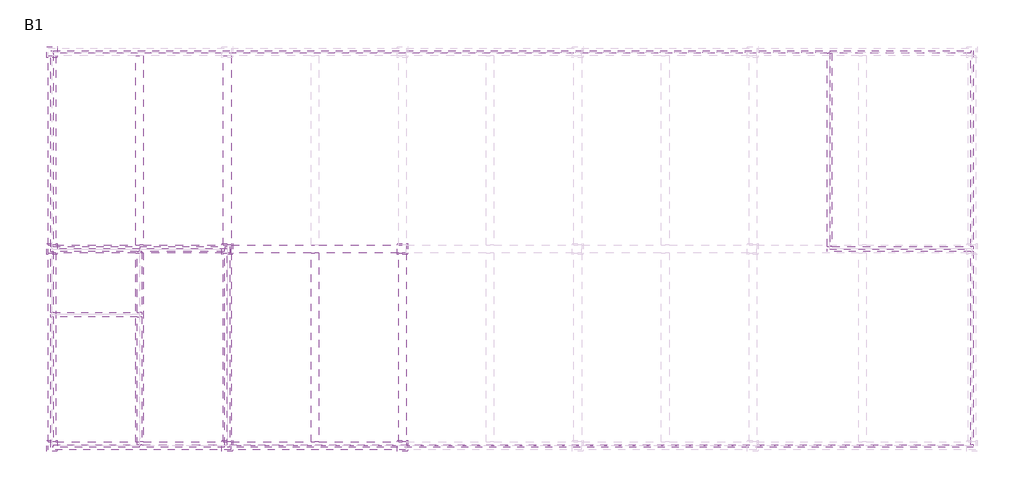
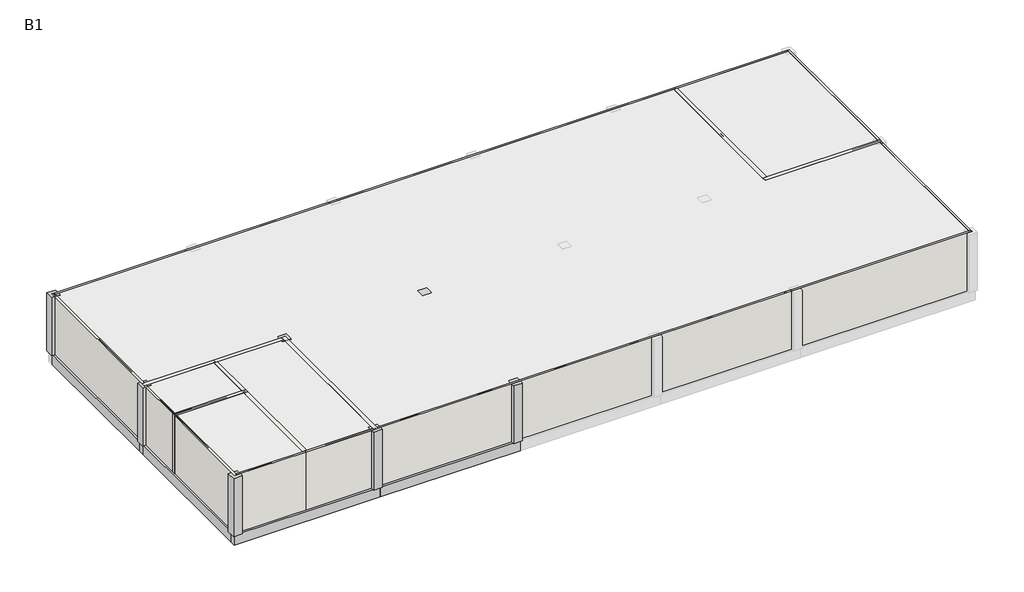
# One storey, part 1 of 2: 18 walls, 12 beams, 7 columns, 5 slabs.
"""IFC4 building model written with IfcOpenShell, lengths in millimetres."""

from ifc_helpers import new_model, si_unit, frame, origin, origin_with_axes, place, context, project, spatial, polyline, outline, extrude, faceted_brep, element, save

model = new_model("IFC4")

# Units and contexts
model_context = context("Model", 3, world=origin())
ifc_project = project(units=[si_unit("LENGTHUNIT", "METRE", prefix="MILLI")], contexts=[model_context])

# Site, building, storey
site = spatial("IfcSite", under=ifc_project)
building = spatial("IfcBuilding", under=site)
storey = spatial("IfcBuildingStorey", under=building, Name="B1", Elevation=-4000.0)

# Beams
placement = place(None, origin())
element("IfcBeam", 1, ObjectType="Concrete-Rectangular-Beam : BM111_400x500_RG1", at=placement, inside=storey, context=model_context, shape_type="SweptSolid", body=[
    extrude(outline(polyline([(49284.6521483, 181748.8614395), (49634.6521483, 181748.8614395), (49634.6521483, 173098.8614395), (49284.6521483, 173098.8614395), (49284.6521483, 181748.8614395)])), frame((0.0, 0.0, -600.0), z_axis=(0.0, 0.0, 1.0), x_axis=(1.0, 0.0, 0.0)), (0.0, 0.0, 1.0), 600.0),
])
element("IfcBeam", 2, ObjectType="Concrete-Rectangular-Beam : BM111_400x500_RG1", at=placement, inside=storey, context=model_context, shape_type="SweptSolid", body=[
    extrude(outline(polyline([(49284.6521483, 172748.8614395), (49634.6521483, 172748.8614395), (49634.6521483, 164098.8614395), (49284.6521483, 164098.8614395), (49284.6521483, 172748.8614395)])), frame((0.0, 0.0, -600.0), z_axis=(0.0, 0.0, 1.0), x_axis=(1.0, 0.0, 0.0)), (0.0, 0.0, 1.0), 600.0),
])
element("IfcBeam", 3, ObjectType="Concrete-Rectangular-Beam : BM111_400x500_RG1", at=placement, inside=storey, context=model_context, shape_type="SweptSolid", body=[
    extrude(outline(polyline([(57284.6521483, 172748.8614395), (57634.6521483, 172748.8614395), (57634.6521483, 164098.8614395), (57284.6521483, 164098.8614395), (57284.6521483, 172748.8614395)])), frame((0.0, 0.0, -600.0), z_axis=(0.0, 0.0, 1.0), x_axis=(1.0, 0.0, 0.0)), (0.0, 0.0, 1.0), 600.0),
])
element("IfcBeam", 4, ObjectType="Concrete-Rectangular-Beam : BM111_400x500_RG1", at=placement, inside=storey, context=model_context, shape_type="Brep", body=[
    faceted_brep([(53634.6521483, 172748.8614395, 0.0), (53634.6521483, 173098.8614395, 0.0), (53284.6521483, 173098.8614395, 0.0), (49634.6521483, 173098.8614395, 0.0), (49284.6521483, 173098.8614395, 0.0), (45634.6521483, 173098.8614395, 0.0), (45284.6521483, 173098.8614395, 0.0), (45284.6521483, 172748.8614395, 0.0), (45634.6521483, 172748.8614395, 0.0), (49284.6521483, 172748.8614395, 0.0), (49634.6521483, 172748.8614395, 0.0), (53284.6521483, 172748.8614395, 0.0), (53634.6521483, 172748.8614395, -600.0), (45284.6521483, 172748.8614395, -600.0), (45634.6521483, 172748.8614395, -600.0), (49284.6521483, 172748.8614395, -600.0), (49634.6521483, 172748.8614395, -600.0), (53284.6521483, 172748.8614395, -600.0), (53634.6521483, 173098.8614395, -600.0), (45284.6521483, 173098.8614395, -600.0), (45634.6521483, 173098.8614395, -600.0), (49284.6521483, 173098.8614395, -600.0), (49634.6521483, 173098.8614395, -600.0), (53284.6521483, 173098.8614395, -600.0)], [[[0, 1, 2, 3, 4, 5, 6, 7, 8, 9, 10, 11]], [[12, 0, 11, 10, 9, 8, 7, 13, 14, 15, 16, 17]], [[18, 12, 17, 16, 15, 14, 13, 19, 20, 21, 22, 23]], [[1, 18, 23, 22, 21, 20, 19, 6, 5, 4, 3, 2]], [[1, 0, 12, 18]], [[7, 6, 19, 13]]]),
])
element("IfcBeam", 5, ObjectType="Concrete-Rectangular-Beam : BM111_400x500_RG1", at=placement, inside=storey, context=model_context, shape_type="Brep", body=[
    faceted_brep([(61634.6521483, 172748.8614395, 0.0), (61634.6521483, 173098.8614395, 0.0), (61284.6521483, 173098.8614395, 0.0), (57634.6521483, 173098.8614395, 0.0), (57284.6521483, 173098.8614395, 0.0), (53634.6521483, 173098.8614395, 0.0), (53634.6521483, 172748.8614395, 0.0), (57284.6521483, 172748.8614395, 0.0), (57634.6521483, 172748.8614395, 0.0), (61284.6521483, 172748.8614395, 0.0), (61634.6521483, 172748.8614395, -600.0), (53634.6521483, 172748.8614395, -600.0), (57284.6521483, 172748.8614395, -600.0), (57634.6521483, 172748.8614395, -600.0), (61284.6521483, 172748.8614395, -600.0), (61634.6521483, 173098.8614395, -600.0), (53634.6521483, 173098.8614395, -600.0), (57284.6521483, 173098.8614395, -600.0), (57634.6521483, 173098.8614395, -600.0), (61284.6521483, 173098.8614395, -600.0)], [[[0, 1, 2, 3, 4, 5, 6, 7, 8, 9]], [[10, 0, 9, 8, 7, 6, 11, 12, 13, 14]], [[15, 10, 14, 13, 12, 11, 16, 17, 18, 19]], [[1, 15, 19, 18, 17, 16, 5, 4, 3, 2]], [[1, 0, 10, 15]], [[6, 5, 16, 11]]]),
])
element("IfcBeam", 6, ObjectType="Concrete-Rectangular-Beam : BM111_400x500_RG1", at=placement, inside=storey, context=model_context, shape_type="Brep", body=[
    faceted_brep([(53634.6521483, 163748.8614395, 0.0), (53634.6521483, 164098.8614395, 0.0), (53284.6521483, 164098.8614395, 0.0), (49634.6521483, 164098.8614395, 0.0), (49284.6521483, 164098.8614395, 0.0), (45634.6521483, 164098.8614395, 0.0), (45284.6521483, 164098.8614395, 0.0), (45284.6521483, 163748.8614395, 0.0), (53634.6521483, 163748.8614395, -600.0), (45284.6521483, 163748.8614395, -600.0), (53634.6521483, 164098.8614395, -600.0), (45284.6521483, 164098.8614395, -600.0), (45634.6521483, 164098.8614395, -600.0), (49284.6521483, 164098.8614395, -600.0), (49634.6521483, 164098.8614395, -600.0), (53284.6521483, 164098.8614395, -600.0)], [[[0, 1, 2, 3, 4, 5, 6, 7]], [[8, 0, 7, 9]], [[10, 8, 9, 11, 12, 13, 14, 15]], [[1, 10, 15, 14, 13, 12, 11, 6, 5, 4, 3, 2]], [[1, 0, 8, 10]], [[7, 6, 11, 9]]]),
])
element("IfcBeam", 7, ObjectType="Concrete-Rectangular-Beam : BM111_400x500_RG1", at=placement, inside=storey, context=model_context, shape_type="Brep", body=[
    faceted_brep([(61634.6521483, 163748.8614395, 0.0), (61634.6521483, 164098.8614395, 0.0), (61284.6521483, 164098.8614395, 0.0), (57634.6521483, 164098.8614395, 0.0), (57284.6521483, 164098.8614395, 0.0), (53634.6521483, 164098.8614395, 0.0), (53634.6521483, 163748.8614395, 0.0), (61634.6521483, 163748.8614395, -600.0), (53634.6521483, 163748.8614395, -600.0), (61634.6521483, 164098.8614395, -600.0), (53634.6521483, 164098.8614395, -600.0), (57284.6521483, 164098.8614395, -600.0), (57634.6521483, 164098.8614395, -600.0), (61284.6521483, 164098.8614395, -600.0)], [[[0, 1, 2, 3, 4, 5, 6]], [[7, 0, 6, 8]], [[9, 7, 8, 10, 11, 12, 13]], [[1, 9, 13, 12, 11, 10, 5, 4, 3, 2]], [[1, 0, 7, 9]], [[6, 5, 10, 8]]]),
])
element("IfcBeam", 8, ObjectType="Concrete-Rectangular-Beam : BM111_400x500_RG1", at=placement, inside=storey, context=model_context, shape_type="SweptSolid", body=[
    extrude(outline(polyline([(45284.6521483, 181748.8614395), (45634.6521483, 181748.8614395), (45634.6521483, 173098.8614395), (45284.6521483, 173098.8614395), (45284.6521483, 181748.8614395)])), frame((0.0, 0.0, -600.0), z_axis=(0.0, 0.0, 1.0), x_axis=(1.0, 0.0, 0.0)), (0.0, 0.0, 1.0), 600.0),
])
element("IfcBeam", 9, ObjectType="Concrete-Rectangular-Beam : BM111_400x500_RG1", at=placement, inside=storey, context=model_context, shape_type="SweptSolid", body=[
    extrude(outline(polyline([(45284.6521483, 172748.8614395), (45634.6521483, 172748.8614395), (45634.6521483, 164098.8614395), (45284.6521483, 164098.8614395), (45284.6521483, 172748.8614395)])), frame((0.0, 0.0, -600.0), z_axis=(0.0, 0.0, 1.0), x_axis=(1.0, 0.0, 0.0)), (0.0, 0.0, 1.0), 600.0),
])
element("IfcBeam", 10, ObjectType="Concrete-Rectangular-Beam : BM111_400x500_RG1", at=placement, inside=storey, context=model_context, shape_type="SweptSolid", body=[
    extrude(outline(polyline([(53284.6521483, 181748.8614395), (53634.6521483, 181748.8614395), (53634.6521483, 173098.8614395), (53284.6521483, 173098.8614395), (53284.6521483, 181748.8614395)])), frame((0.0, 0.0, -600.0), z_axis=(0.0, 0.0, 1.0), x_axis=(1.0, 0.0, 0.0)), (0.0, 0.0, 1.0), 600.0),
])
element("IfcBeam", 11, ObjectType="Concrete-Rectangular-Beam : BM111_400x500_RG1", at=placement, inside=storey, context=model_context, shape_type="SweptSolid", body=[
    extrude(outline(polyline([(53284.6521483, 172748.8614395), (53634.6521483, 172748.8614395), (53634.6521483, 164098.8614395), (53284.6521483, 164098.8614395), (53284.6521483, 172748.8614395)])), frame((0.0, 0.0, -600.0), z_axis=(0.0, 0.0, 1.0), x_axis=(1.0, 0.0, 0.0)), (0.0, 0.0, 1.0), 600.0),
])
element("IfcBeam", 12, ObjectType="Concrete-Rectangular-Beam : BM111_400x500_RG1", at=placement, inside=storey, context=model_context, shape_type="SweptSolid", body=[
    extrude(outline(polyline([(61284.6521483, 172748.8614395), (61634.6521483, 172748.8614395), (61634.6521483, 164098.8614395), (61284.6521483, 164098.8614395), (61284.6521483, 172748.8614395)])), frame((0.0, 0.0, -600.0), z_axis=(0.0, 0.0, 1.0), x_axis=(1.0, 0.0, 0.0)), (0.0, 0.0, 1.0), 600.0),
])

# Columns
element("IfcColumn", 13, ObjectType="Concrete-Rectangular-Column : CL111_500x500", at=placement, inside=storey, context=model_context, shape_type="Brep", body=[
    faceted_brep([(45709.6521483, 182173.8614395, 0.0), (45709.6521483, 181673.8614395, 0.0), (45209.6521483, 181673.8614395, 0.0), (45209.6521483, 182173.8614395, 0.0), (45709.6521483, 182173.8614395, 3500.0), (45709.6521483, 182098.8614395, 3500.0), (45709.6521483, 181748.8614395, 3500.0), (45709.6521483, 181673.8614395, 3500.0), (45634.6521483, 181673.8614395, 3500.0), (45284.6521483, 181673.8614395, 3500.0), (45209.6521483, 181673.8614395, 3500.0), (45209.6521483, 182173.8614395, 3500.0)], [[[0, 1, 2, 3]], [[4, 5, 6, 7, 1, 0]], [[7, 8, 9, 10, 2, 1]], [[10, 11, 3, 2]], [[11, 4, 0, 3]], [[4, 11, 10, 9, 8, 7, 6, 5]]]),
])
element("IfcColumn", 14, ObjectType="Concrete-Rectangular-Column : CL111_500x500", at=placement, inside=storey, context=model_context, shape_type="Brep", body=[
    faceted_brep([(45709.6521483, 173173.8614395, 0.0), (45709.6521483, 172673.8614395, 0.0), (45209.6521483, 172673.8614395, 0.0), (45209.6521483, 173173.8614395, 0.0), (45709.6521483, 173173.8614395, 3500.0), (45709.6521483, 173098.8614395, 3500.0), (45709.6521483, 172748.8614395, 3500.0), (45709.6521483, 172673.8614395, 3500.0), (45634.6521483, 172673.8614395, 3500.0), (45284.6521483, 172673.8614395, 3500.0), (45209.6521483, 172673.8614395, 3500.0), (45209.6521483, 173173.8614395, 3500.0), (45284.6521483, 173173.8614395, 3500.0), (45634.6521483, 173173.8614395, 3500.0)], [[[0, 1, 2, 3]], [[4, 5, 6, 7, 1, 0]], [[7, 8, 9, 10, 2, 1]], [[10, 11, 3, 2]], [[11, 12, 13, 4, 0, 3]], [[4, 13, 12, 11, 10, 9, 8, 7, 6, 5]]]),
])
element("IfcColumn", 15, ObjectType="Concrete-Rectangular-Column : CL111_500x500", at=placement, inside=storey, context=model_context, shape_type="Brep", body=[
    faceted_brep([(53709.6521483, 173173.8614395, 0.0), (53709.6521483, 172673.8614395, 0.0), (53209.6521483, 172673.8614395, 0.0), (53209.6521483, 173173.8614395, 0.0), (53709.6521483, 173173.8614395, 3500.0), (53709.6521483, 173098.8614395, 3500.0), (53709.6521483, 172748.8614395, 3500.0), (53709.6521483, 172673.8614395, 3500.0), (53634.6521483, 172673.8614395, 3500.0), (53284.6521483, 172673.8614395, 3500.0), (53209.6521483, 172673.8614395, 3500.0), (53209.6521483, 172748.8614395, 3500.0), (53209.6521483, 173098.8614395, 3500.0), (53209.6521483, 173173.8614395, 3500.0), (53284.6521483, 173173.8614395, 3500.0), (53634.6521483, 173173.8614395, 3500.0)], [[[0, 1, 2, 3]], [[4, 5, 6, 7, 1, 0]], [[7, 8, 9, 10, 2, 1]], [[10, 11, 12, 13, 3, 2]], [[13, 14, 15, 4, 0, 3]], [[4, 15, 14, 13, 12, 11, 10, 9, 8, 7, 6, 5]]]),
])
element("IfcColumn", 16, ObjectType="Concrete-Rectangular-Column : CL111_500x500", at=placement, inside=storey, context=model_context, shape_type="Brep", body=[
    faceted_brep([(61709.6521483, 173173.8614395, 0.0), (61709.6521483, 172673.8614395, 0.0), (61209.6521483, 172673.8614395, 0.0), (61209.6521483, 173173.8614395, 0.0), (61709.6521483, 173173.8614395, 3500.0), (61709.6521483, 173098.8614395, 3500.0), (61709.6521483, 172748.8614395, 3500.0), (61709.6521483, 172673.8614395, 3500.0), (61634.6521483, 172673.8614395, 3500.0), (61284.6521483, 172673.8614395, 3500.0), (61209.6521483, 172673.8614395, 3500.0), (61209.6521483, 172748.8614395, 3500.0), (61209.6521483, 173098.8614395, 3500.0), (61209.6521483, 173173.8614395, 3500.0), (61284.6521483, 173173.8614395, 3500.0), (61634.6521483, 173173.8614395, 3500.0)], [[[0, 1, 2, 3]], [[4, 5, 6, 7, 1, 0]], [[7, 8, 9, 10, 2, 1]], [[10, 11, 12, 13, 3, 2]], [[13, 14, 15, 4, 0, 3]], [[4, 15, 14, 13, 12, 11, 10, 9, 8, 7, 6, 5]]]),
])
element("IfcColumn", 17, ObjectType="Concrete-Rectangular-Column : CL111_500x500", at=placement, inside=storey, context=model_context, shape_type="Brep", body=[
    faceted_brep([(45709.6521483, 164173.8614395, 0.0), (45709.6521483, 163673.8614395, 0.0), (45209.6521483, 163673.8614395, 0.0), (45209.6521483, 164173.8614395, 0.0), (45709.6521483, 164173.8614395, 3500.0), (45709.6521483, 164098.8614395, 3500.0), (45709.6521483, 163748.8614395, 3500.0), (45709.6521483, 163673.8614395, 3500.0), (45209.6521483, 163673.8614395, 3500.0), (45209.6521483, 164173.8614395, 3500.0), (45284.6521483, 164173.8614395, 3500.0), (45634.6521483, 164173.8614395, 3500.0)], [[[0, 1, 2, 3]], [[4, 5, 6, 7, 1, 0]], [[7, 8, 2, 1]], [[8, 9, 3, 2]], [[9, 10, 11, 4, 0, 3]], [[4, 11, 10, 9, 8, 7, 6, 5]]]),
])
element("IfcColumn", 18, ObjectType="Concrete-Rectangular-Column : CL111_500x500", at=placement, inside=storey, context=model_context, shape_type="Brep", body=[
    faceted_brep([(53709.6521483, 164173.8614395, 0.0), (53709.6521483, 163673.8614395, 0.0), (53209.6521483, 163673.8614395, 0.0), (53209.6521483, 164173.8614395, 0.0), (53709.6521483, 164173.8614395, 3500.0), (53709.6521483, 164098.8614395, 3500.0), (53709.6521483, 163748.8614395, 3500.0), (53709.6521483, 163673.8614395, 3500.0), (53209.6521483, 163673.8614395, 3500.0), (53209.6521483, 163748.8614395, 3500.0), (53209.6521483, 164098.8614395, 3500.0), (53209.6521483, 164173.8614395, 3500.0), (53284.6521483, 164173.8614395, 3500.0), (53634.6521483, 164173.8614395, 3500.0)], [[[0, 1, 2, 3]], [[4, 5, 6, 7, 1, 0]], [[7, 8, 2, 1]], [[8, 9, 10, 11, 3, 2]], [[11, 12, 13, 4, 0, 3]], [[4, 13, 12, 11, 10, 9, 8, 7, 6, 5]]]),
])
element("IfcColumn", 19, ObjectType="Concrete-Rectangular-Column : CL111_500x500", at=placement, inside=storey, context=model_context, shape_type="Brep", body=[
    faceted_brep([(61709.6521483, 164173.8614395, 0.0), (61709.6521483, 163673.8614395, 0.0), (61209.6521483, 163673.8614395, 0.0), (61209.6521483, 164173.8614395, 0.0), (61709.6521483, 164173.8614395, 3500.0), (61709.6521483, 164098.8614395, 3500.0), (61709.6521483, 163748.8614395, 3500.0), (61709.6521483, 163673.8614395, 3500.0), (61209.6521483, 163673.8614395, 3500.0), (61209.6521483, 163748.8614395, 3500.0), (61209.6521483, 164098.8614395, 3500.0), (61209.6521483, 164173.8614395, 3500.0), (61284.6521483, 164173.8614395, 3500.0), (61634.6521483, 164173.8614395, 3500.0)], [[[0, 1, 2, 3]], [[4, 5, 6, 7, 1, 0]], [[7, 8, 2, 1]], [[8, 9, 10, 11, 3, 2]], [[11, 12, 13, 4, 0, 3]], [[4, 13, 12, 11, 10, 9, 8, 7, 6, 5]]]),
])

# Slabs
element("IfcSlab", 20, ObjectType="CFS11_Slab RC_T150", at=placement, inside=storey, context=model_context, shape_type="SweptSolid", body=[
    extrude(outline(polyline([(87459.6521483, 181923.8614395), (87459.6521483, 172923.8614395), (80959.6521483, 172923.8614395), (80959.6521483, 181923.8614395), (87459.6521483, 181923.8614395)])), frame((0.0, 0.0, -150.0), z_axis=(0.0, 0.0, 1.0), x_axis=(1.0, 0.0, 0.0)), (0.0, 0.0, 1.0), 150.0),
])
element("IfcSlab", 21, ObjectType="CFS11_Slab RC_T150", at=placement, inside=storey, context=model_context, shape_type="SweptSolid", body=[
    extrude(outline(polyline([(53459.6521483, 163923.8614395), (49459.6521483, 163923.8614395), (49459.6521483, 172923.8614395), (53459.6521483, 172923.8614395), (53459.6521483, 163923.8614395)])), frame((0.0, 0.0, -150.0), z_axis=(0.0, 0.0, 1.0), x_axis=(1.0, 0.0, 0.0)), (0.0, 0.0, 1.0), 150.0),
])
element("IfcSlab", 22, ObjectType="CFS11_Slab RC_T150", at=placement, inside=storey, context=model_context, shape_type="SweptSolid", body=[
    extrude(outline(polyline([(80959.6521483, 181923.8614395), (80959.6521483, 172923.8614395), (87459.6521483, 172923.8614395), (87459.6521483, 163923.8614395), (53459.6521483, 163923.8614395), (53459.6521483, 172923.8614395), (45459.6521483, 172923.8614395), (45459.6521483, 181923.8614395), (80959.6521483, 181923.8614395)])), frame((0.0, 0.0, -150.0), z_axis=(0.0, 0.0, 1.0), x_axis=(1.0, 0.0, 0.0)), (0.0, 0.0, 1.0), 150.0),
])
element("IfcSlab", 23, ObjectType="CFS11_Slab RC_T150", at=placement, inside=storey, context=model_context, shape_type="SweptSolid", body=[
    extrude(outline(polyline([(45459.6521483, 163923.8614395), (45459.6521483, 169923.8614395), (49459.6521483, 169923.8614395), (49459.6521483, 163923.8614395), (45459.6521483, 163923.8614395)])), frame((0.0, 0.0, -150.0), z_axis=(0.0, 0.0, 1.0), x_axis=(1.0, 0.0, 0.0)), (0.0, 0.0, 1.0), 150.0),
])
element("IfcSlab", 24, ObjectType="CFS11_Slab RC_T150", at=placement, inside=storey, context=model_context, shape_type="SweptSolid", body=[
    extrude(outline(polyline([(45459.6521483, 172923.8614395), (49459.6521483, 172923.8614395), (49459.6521483, 169923.8614395), (45459.6521483, 169923.8614395), (45459.6521483, 172923.8614395)])), frame((0.0, 0.0, -150.0), z_axis=(0.0, 0.0, 1.0), x_axis=(1.0, 0.0, 0.0)), (0.0, 0.0, 1.0), 150.0),
])

# Walls
element("IfcWall", 25, ObjectType="WA211_Exterior-Cement Brick-90mm", at=placement, inside=storey, context=model_context, shape_type="Brep", body=[
    faceted_brep([(80959.6521483, 181866.8614395, 0.0), (81066.6521483, 181866.8614395, 0.0), (87402.6521483, 181866.8614395, 0.0), (87402.6521483, 181866.8614395, 3500.0), (81066.6521483, 181866.8614395, 3500.0), (80959.6521483, 181866.8614395, 3500.0), (80959.6521483, 181980.8614395, 0.0), (80959.6521483, 181980.8614395, 3500.0), (87402.6521483, 181980.8614395, 3500.0), (87402.6521483, 181980.8614395, 0.0)], [[[0, 1, 2, 3, 4, 5]], [[6, 7, 8, 9]], [[2, 1, 0, 6, 9]], [[5, 4, 3, 8, 7]], [[0, 5, 7, 6]], [[3, 2, 9, 8]]]),
])
element("IfcWall", 26, ObjectType="WA211_Exterior-Cement Brick-90mm", at=placement, inside=storey, context=model_context, shape_type="Brep", body=[
    faceted_brep([(87402.6521483, 181980.8614395, 0.0), (87402.6521483, 181866.8614395, 0.0), (87402.6521483, 173030.8614395, 0.0), (87402.6521483, 173030.8614395, 3500.0), (87402.6521483, 181866.8614395, 3500.0), (87402.6521483, 181980.8614395, 3500.0), (87516.6521483, 181980.8614395, 0.0), (87516.6521483, 181980.8614395, 3500.0), (87516.6521483, 173030.8614395, 3500.0), (87516.6521483, 173030.8614395, 0.0)], [[[0, 1, 2, 3, 4, 5]], [[6, 7, 8, 9]], [[2, 1, 0, 6, 9]], [[5, 4, 3, 8, 7]], [[0, 5, 7, 6]], [[3, 2, 9, 8]]]),
])
element("IfcWall", 27, ObjectType="WA211_Exterior-Cement Brick-90mm", at=placement, inside=storey, context=model_context, shape_type="Brep", body=[
    faceted_brep([(53352.6521483, 163980.8614395, 0.0), (49566.6521483, 163980.8614395, 0.0), (49459.6521483, 163980.8614395, 0.0), (49459.6521483, 163980.8614395, 3500.0), (49566.6521483, 163980.8614395, 3500.0), (53352.6521483, 163980.8614395, 3500.0), (53352.6521483, 163866.8614395, 0.0), (53352.6521483, 163866.8614395, 3500.0), (49459.6521483, 163866.8614395, 3500.0), (49459.6521483, 163866.8614395, 0.0)], [[[0, 1, 2, 3, 4, 5]], [[6, 7, 8, 9]], [[2, 1, 0, 6, 9]], [[3, 2, 9, 8]], [[5, 4, 3, 8, 7]], [[0, 5, 7, 6]]]),
])
element("IfcWall", 28, ObjectType="WA211_Exterior-Cement Brick-90mm", at=placement, inside=storey, context=model_context, shape_type="Brep", body=[
    faceted_brep([(45516.6521483, 173030.8614395, 0.0), (45516.6521483, 181866.8614395, 0.0), (45516.6521483, 181980.8614395, 0.0), (45516.6521483, 181980.8614395, 3500.0), (45516.6521483, 181866.8614395, 3500.0), (45516.6521483, 173030.8614395, 3500.0), (45402.6521483, 173030.8614395, 0.0), (45402.6521483, 173030.8614395, 3500.0), (45402.6521483, 181980.8614395, 3500.0), (45402.6521483, 181980.8614395, 0.0)], [[[0, 1, 2, 3, 4, 5]], [[6, 7, 8, 9]], [[2, 1, 0, 6, 9]], [[5, 4, 3, 8, 7]], [[3, 2, 9, 8]], [[0, 5, 7, 6]]]),
])
element("IfcWall", 29, ObjectType="WA211_Exterior-Cement Brick-90mm", at=placement, inside=storey, context=model_context, shape_type="Brep", body=[
    faceted_brep([(87516.6521483, 163980.8614395, 0.0), (87402.6521483, 163980.8614395, 0.0), (53566.6521483, 163980.8614395, 0.0), (53566.6521483, 163980.8614395, 3500.0), (87402.6521483, 163980.8614395, 3500.0), (87516.6521483, 163980.8614395, 3500.0), (87516.6521483, 163866.8614395, 0.0), (87516.6521483, 163866.8614395, 3500.0), (53566.6521483, 163866.8614395, 3500.0), (53566.6521483, 163866.8614395, 0.0)], [[[0, 1, 2, 3, 4, 5]], [[6, 7, 8, 9]], [[2, 1, 0, 6, 9]], [[5, 4, 3, 8, 7]], [[0, 5, 7, 6]], [[3, 2, 9, 8]]]),
])
element("IfcWall", 30, ObjectType="WA211_Exterior-Cement Brick-90mm", at=placement, inside=storey, context=model_context, shape_type="SweptSolid", body=[
    extrude(outline(polyline([(87402.6521483, 163980.8614395), (87402.6521483, 172816.8614395), (87516.6521483, 172816.8614395), (87516.6521483, 163980.8614395), (87402.6521483, 163980.8614395)])), origin_with_axes(), (0.0, 0.0, 1.0), 3500.0),
])
element("IfcWall", 31, ObjectType="WA211_Exterior-Cement Brick-90mm", at=placement, inside=storey, context=model_context, shape_type="Brep", body=[
    faceted_brep([(45516.6521483, 181866.8614395, 0.0), (80852.6521483, 181866.8614395, 0.0), (80959.6521483, 181866.8614395, 0.0), (80959.6521483, 181866.8614395, 3500.0), (80852.6521483, 181866.8614395, 3500.0), (45516.6521483, 181866.8614395, 3500.0), (45516.6521483, 181980.8614395, 0.0), (45516.6521483, 181980.8614395, 3500.0), (80959.6521483, 181980.8614395, 3500.0), (80959.6521483, 181980.8614395, 0.0)], [[[0, 1, 2, 3, 4, 5]], [[6, 7, 8, 9]], [[2, 1, 0, 6, 9]], [[3, 2, 9, 8]], [[5, 4, 3, 8, 7]], [[0, 5, 7, 6]]]),
])
element("IfcWall", 32, ObjectType="WA211_Exterior-Cement Brick-90mm", at=placement, inside=storey, context=model_context, shape_type="Brep", body=[
    faceted_brep([(49459.6521483, 163980.8614395, 0.0), (49352.6521483, 163980.8614395, 0.0), (45516.6521483, 163980.8614395, 0.0), (45516.6521483, 163980.8614395, 3500.0), (49352.6521483, 163980.8614395, 3500.0), (49459.6521483, 163980.8614395, 3500.0), (49459.6521483, 163866.8614395, 0.0), (49459.6521483, 163866.8614395, 3500.0), (45516.6521483, 163866.8614395, 3500.0), (45516.6521483, 163866.8614395, 0.0)], [[[0, 1, 2, 3, 4, 5]], [[6, 7, 8, 9]], [[2, 1, 0, 6, 9]], [[5, 4, 3, 8, 7]], [[0, 5, 7, 6]], [[3, 2, 9, 8]]]),
])
element("IfcWall", 33, ObjectType="WA211_Exterior-Cement Brick-90mm", at=placement, inside=storey, context=model_context, shape_type="Brep", body=[
    faceted_brep([(45516.6521483, 163866.8614395, 0.0), (45516.6521483, 163980.8614395, 0.0), (45516.6521483, 169816.8614395, 0.0), (45516.6521483, 169816.8614395, 3500.0), (45516.6521483, 163980.8614395, 3500.0), (45516.6521483, 163866.8614395, 3500.0), (45402.6521483, 163866.8614395, 0.0), (45402.6521483, 163866.8614395, 3500.0), (45402.6521483, 169816.8614395, 3500.0), (45402.6521483, 169816.8614395, 0.0)], [[[0, 1, 2, 3, 4, 5]], [[6, 7, 8, 9]], [[2, 1, 0, 6, 9]], [[5, 4, 3, 8, 7]], [[0, 5, 7, 6]], [[3, 2, 9, 8]]]),
])
element("IfcWall", 34, ObjectType="WA211_Exterior-Cement Brick-90mm", at=placement, inside=storey, context=model_context, shape_type="SweptSolid", body=[
    extrude(outline(polyline([(45516.6521483, 172816.8614395), (45516.6521483, 170030.8614395), (45402.6521483, 170030.8614395), (45402.6521483, 172816.8614395), (45516.6521483, 172816.8614395)])), origin_with_axes(), (0.0, 0.0, 1.0), 3500.0),
])
element("IfcWall", 35, ObjectType="WA221_Interior-Cement Block-190mm", at=placement, inside=storey, context=model_context, shape_type="Brep", body=[
    faceted_brep([(80852.6521483, 181866.8614395, 0.0), (80852.6521483, 173030.8614395, 0.0), (80852.6521483, 173030.8614395, 3500.0), (80852.6521483, 181866.8614395, 3500.0), (81066.6521483, 181866.8614395, 0.0), (81066.6521483, 181866.8614395, 3500.0), (81066.6521483, 173030.8614395, 3500.0), (81066.6521483, 173030.8614395, 0.0), (80959.6521483, 181866.8614395, 0.0), (80959.6521483, 181866.8614395, 3500.0)], [[[0, 1, 2, 3]], [[4, 5, 6, 7]], [[1, 0, 8, 4, 7]], [[3, 2, 6, 5, 9]], [[0, 3, 9, 5, 4, 8]], [[2, 1, 7, 6]]]),
])
element("IfcWall", 36, ObjectType="WA221_Interior-Cement Block-190mm", at=placement, inside=storey, context=model_context, shape_type="Brep", body=[
    faceted_brep([(87516.6521483, 173030.8614395, 0.0), (87402.6521483, 173030.8614395, 0.0), (81066.6521483, 173030.8614395, 0.0), (80852.6521483, 173030.8614395, 0.0), (80852.6521483, 173030.8614395, 3500.0), (81066.6521483, 173030.8614395, 3500.0), (87402.6521483, 173030.8614395, 3500.0), (87516.6521483, 173030.8614395, 3500.0), (87516.6521483, 172816.8614395, 0.0), (87516.6521483, 172816.8614395, 3500.0), (87402.6521483, 172816.8614395, 3500.0), (80852.6521483, 172816.8614395, 3500.0), (80852.6521483, 172816.8614395, 0.0), (87402.6521483, 172816.8614395, 0.0)], [[[0, 1, 2, 3, 4, 5, 6, 7]], [[8, 9, 10, 11, 12, 13]], [[3, 2, 1, 0, 8, 13, 12]], [[7, 6, 5, 4, 11, 10, 9]], [[4, 3, 12, 11]], [[0, 7, 9, 8]]]),
])
element("IfcWall", 37, ObjectType="WA221_Interior-Cement Block-190mm", at=placement, inside=storey, context=model_context, shape_type="Brep", body=[
    faceted_brep([(53566.6521483, 163866.8614395, 0.0), (53566.6521483, 163980.8614395, 0.0), (53566.6521483, 173030.8614395, 0.0), (53566.6521483, 173030.8614395, 3500.0), (53566.6521483, 163980.8614395, 3500.0), (53566.6521483, 163866.8614395, 3500.0), (53352.6521483, 163866.8614395, 0.0), (53352.6521483, 163866.8614395, 3500.0), (53352.6521483, 163980.8614395, 3500.0), (53352.6521483, 172816.8614395, 3500.0), (53352.6521483, 173030.8614395, 3500.0), (53352.6521483, 173030.8614395, 0.0), (53352.6521483, 172816.8614395, 0.0), (53352.6521483, 163980.8614395, 0.0)], [[[0, 1, 2, 3, 4, 5]], [[6, 7, 8, 9, 10, 11, 12, 13]], [[2, 1, 0, 6, 13, 12, 11]], [[5, 4, 3, 10, 9, 8, 7]], [[3, 2, 11, 10]], [[0, 5, 7, 6]]]),
])
element("IfcWall", 38, ObjectType="WA221_Interior-Cement Block-190mm", at=placement, inside=storey, context=model_context, shape_type="Brep", body=[
    faceted_brep([(49459.6521483, 172816.8614395, 0.0), (49566.6521483, 172816.8614395, 0.0), (53352.6521483, 172816.8614395, 0.0), (53352.6521483, 172816.8614395, 3500.0), (49566.6521483, 172816.8614395, 3500.0), (49459.6521483, 172816.8614395, 3500.0), (49459.6521483, 173030.8614395, 0.0), (49459.6521483, 173030.8614395, 3500.0), (53352.6521483, 173030.8614395, 3500.0), (53352.6521483, 173030.8614395, 0.0)], [[[0, 1, 2, 3, 4, 5]], [[6, 7, 8, 9]], [[2, 1, 0, 6, 9]], [[5, 4, 3, 8, 7]], [[0, 5, 7, 6]], [[3, 2, 9, 8]]]),
])
element("IfcWall", 39, ObjectType="WA221_Interior-Cement Block-190mm", at=placement, inside=storey, context=model_context, shape_type="Brep", body=[
    faceted_brep([(49352.6521483, 169816.8614395, 0.0), (49352.6521483, 163980.8614395, 0.0), (49352.6521483, 163980.8614395, 3500.0), (49352.6521483, 169816.8614395, 3500.0), (49566.6521483, 169816.8614395, 0.0), (49566.6521483, 169816.8614395, 3500.0), (49566.6521483, 163980.8614395, 3500.0), (49566.6521483, 163980.8614395, 0.0), (49459.6521483, 163980.8614395, 0.0), (49459.6521483, 163980.8614395, 3500.0)], [[[0, 1, 2, 3]], [[4, 5, 6, 7]], [[1, 0, 4, 7, 8]], [[3, 2, 9, 6, 5]], [[2, 1, 8, 7, 6, 9]], [[0, 3, 5, 4]]]),
])
element("IfcWall", 40, ObjectType="WA221_Interior-Cement Block-190mm", at=placement, inside=storey, context=model_context, shape_type="Brep", body=[
    faceted_brep([(49352.6521483, 172816.8614395, 0.0), (49352.6521483, 170030.8614395, 0.0), (49352.6521483, 170030.8614395, 3500.0), (49352.6521483, 172816.8614395, 3500.0), (49566.6521483, 172816.8614395, 0.0), (49566.6521483, 172816.8614395, 3500.0), (49566.6521483, 170030.8614395, 3500.0), (49566.6521483, 170030.8614395, 0.0), (49459.6521483, 172816.8614395, 0.0), (49459.6521483, 172816.8614395, 3500.0)], [[[0, 1, 2, 3]], [[4, 5, 6, 7]], [[1, 0, 8, 4, 7]], [[3, 2, 6, 5, 9]], [[0, 3, 9, 5, 4, 8]], [[2, 1, 7, 6]]]),
])
element("IfcWall", 41, ObjectType="WA221_Interior-Cement Block-190mm", at=placement, inside=storey, context=model_context, shape_type="Brep", body=[
    faceted_brep([(49459.6521483, 173030.8614395, 0.0), (45516.6521483, 173030.8614395, 0.0), (45402.6521483, 173030.8614395, 0.0), (45402.6521483, 173030.8614395, 3500.0), (45516.6521483, 173030.8614395, 3500.0), (49459.6521483, 173030.8614395, 3500.0), (49459.6521483, 172816.8614395, 0.0), (49459.6521483, 172816.8614395, 3500.0), (49352.6521483, 172816.8614395, 3500.0), (45516.6521483, 172816.8614395, 3500.0), (45402.6521483, 172816.8614395, 3500.0), (45402.6521483, 172816.8614395, 0.0), (45516.6521483, 172816.8614395, 0.0), (49352.6521483, 172816.8614395, 0.0)], [[[0, 1, 2, 3, 4, 5]], [[6, 7, 8, 9, 10, 11, 12, 13]], [[2, 1, 0, 6, 13, 12, 11]], [[5, 4, 3, 10, 9, 8, 7]], [[0, 5, 7, 6]], [[3, 2, 11, 10]]]),
])
element("IfcWall", 42, ObjectType="WA221_Interior-Cement Block-190mm", at=placement, inside=storey, context=model_context, shape_type="Brep", body=[
    faceted_brep([(49566.6521483, 170030.8614395, 0.0), (49352.6521483, 170030.8614395, 0.0), (45516.6521483, 170030.8614395, 0.0), (45402.6521483, 170030.8614395, 0.0), (45402.6521483, 170030.8614395, 3500.0), (45516.6521483, 170030.8614395, 3500.0), (49352.6521483, 170030.8614395, 3500.0), (49566.6521483, 170030.8614395, 3500.0), (49566.6521483, 169816.8614395, 0.0), (49566.6521483, 169816.8614395, 3500.0), (49352.6521483, 169816.8614395, 3500.0), (45516.6521483, 169816.8614395, 3500.0), (45402.6521483, 169816.8614395, 3500.0), (45402.6521483, 169816.8614395, 0.0), (45516.6521483, 169816.8614395, 0.0), (49352.6521483, 169816.8614395, 0.0)], [[[0, 1, 2, 3, 4, 5, 6, 7]], [[8, 9, 10, 11, 12, 13, 14, 15]], [[3, 2, 1, 0, 8, 15, 14, 13]], [[7, 6, 5, 4, 12, 11, 10, 9]], [[0, 7, 9, 8]], [[4, 3, 13, 12]]]),
])

save(model, "model.ifc")

# Revit data of these elements
# Project information
#   Building Name = "MAIN GATE SECURITY BUILDING"
#   Project Status = "Project Status"
#   Client Name = "현대엔지니어링"
#   Project Address = "서울시 종로구 율곡로 75(계동)"
#   Project Name = "Therma Visayas Energy Project"
#   Project Number = "-"
# Grids (mm)
#   "1": line (45459.652, 190234.526) -> (45459.652, 152139.384)
#   "2": line (53459.652, 190234.526) -> (53459.652, 152139.384)
#   "3": line (61459.652, 190234.526) -> (61459.652, 152139.384)
#   "4": line (69459.652, 190234.526) -> (69459.652, 152139.384)
#   "5": line (77459.652, 190234.526) -> (77459.652, 152139.384)
#   "6": line (87459.652, 190234.526) -> (87459.652, 152139.384)
#   "C": line (39389.066, 181923.861) -> (102402.798, 181923.861)
#   "B": line (39389.066, 172923.861) -> (102402.798, 172923.861)
#   "A": line (39389.066, 163923.861) -> (102402.798, 163923.861)
# Type "Concrete-Rectangular-Beam : BM111_400x500_RG1"
#   중앙부 하부근 = "3-D20"
#   중앙부 상부근 = "3-D20"
#   중앙부 보조근 = ""
#   중앙부 늑근 = "2-D10 @200"
#   외단부 하부근 = "3-D20"
#   외단부 상부근 = "3-D20"
#   외단부 보조근 = ""
#   외단부 늑근 = "2-D10 @100"
#   부호 = "RG1"
#   내단부 하부근 = "3-D20"
#   내단부 상부근 = "3-D20"
#   내단부 보조근 = ""
#   내단부 늑근 = "2-D10 @100"
#   ALL 하부근 = ""
#   ALL 상부근 = ""
#   ALL 보조근 = ""
#   ALL 늑근 = ""
#   Width = 400 mm
#   Height = 500 mm
#   Length [instance default] = 1524 mm
#   Structural Material [instance default] = 콘크리트 - 현장타설 콘크리트
#   hec_material3 [instance default] = none
#   hec_material2 [instance default] = none
#   hec_material1 [instance default] = none
#   Assembly Code = ""
# Type "Concrete-Rectangular-Column : CL111_500x500"
#   Description = "UG 철골 기둥용 Pedestal"
#   b = 500 mm
#   h = 500 mm
#   hec_material3 [instance default] = none
#   hec_material2 [instance default] = A03AE056-00001_Bitumen/Bituminous/Asphalt Coating
#   hec_material1 [instance default] = A03AC035-00001_Form Work (3 times in use)_Flat
#   Structural Material [instance default] = A03AC032-00007_Structural Concrete_Type1_25MPa-30Mpa
# Type "CFS11_Slab RC_T150"
#   Keynote = ""
#   Type Comments = "구조_콘크리트"
#   Function = 0
#   Layers, outside or top first: 150 mm "14200-030101_Concrete Pouring" (function 1)
# Type "WA211_Exterior-Cement Brick-90mm"
#   Type Comments = ""
#   Layers, outside or top first: 0 mm "A04AL081-00001_Skirt_Acrylic Emulsion Paint" (function 100); 0 mm "A04AL077-00001_Ext Wall Painting_Acrylic Emulsion Paint" (function 100); 12 mm "A04AS164-00001_Plastering_Ext" (function 4); 90 mm "A04AK073-00001_Concrete Brick_0.5B" (function 1); 12 mm "A04AS164-00002_Plastering_Int" (function 5); 0 mm "A04AL078-00002_Int Wall Painting_Water Emulsion Paint" (function 100); 0 mm "A04AL081-00001_Skirt_Acrylic Emulsion Paint" (function 100)
# Type "WA221_Interior-Cement Block-190mm"
#   Type Comments = ""
#   Layers, outside or top first: 0 mm "A04AL081-00001_Skirt_Acrylic Emulsion Paint" (function 100); 0 mm "A04AL078-00002_Int Wall Painting_Water Emulsion Paint" (function 100); 12 mm "A04AS164-00002_Plastering_Int" (function 2); 190 mm "A04AK069-00002_Reinforced Concrete Block_THK 100-200mm" (function 1); 12 mm "A04AS164-00002_Plastering_Int" (function 2); 0 mm "A04AL078-00002_Int Wall Painting_Water Emulsion Paint" (function 100); 0 mm "A04AL081-00001_Skirt_Acrylic Emulsion Paint" (function 100)
# Elements 1, 2, 3, 4, 5, 6, 7, 8, 9, 10, 11, 12 (IfcBeam, "Concrete-Rectangular-Beam : BM111_400x500_RG1")
#   Comments = ""
#   hec_material3 = none
#   hec_material2 = none
#   hec_material1 = none
#   Structural Material = 콘크리트 - 현장타설 콘크리트
#   Phase Created = New Construction
#   Materials on its faces: "콘크리트 - 현장타설 콘크리트"
# Elements 13, 14, 15, 16, 17, 18, 19 (IfcColumn, "Concrete-Rectangular-Column : CL111_500x500")
#   Comments = ""
#   hec_material3 = none
#   hec_material2 = none
#   hec_material1 = none
#   Structural Material = 콘크리트 - 현장타설 콘크리트
#   Phase Created = New Construction
#   Materials on its faces: "콘크리트 - 현장타설 콘크리트"
# Elements 20, 21, 22, 23, 24 (IfcSlab, "CFS11_Slab RC_T150")
#   Height Offset From Level = 0 mm
#   Phase Created = New Construction
#   Materials on its faces: "14200-030101_Concrete Pouring"
# Elements 25, 27, 30, 31, 32, 34 (IfcWall, "WA211_Exterior-Cement Brick-90mm")
#   Top Offset = 0 mm
#   Base Offset = 0 mm
#   Unconnected Height = 3500 mm
#   wall height = 3500 mm
#   Phase Created = New Construction
#   Base Constraint = GF
#   Materials on its faces: "Default Wall", "A04AS164-00002_Plastering_Int", "A04AS164-00001_Plastering_Ext"
# Elements 26, 28, 29, 33 (IfcWall, "WA211_Exterior-Cement Brick-90mm")
#   Top Offset = 0 mm
#   Base Offset = 0 mm
#   Unconnected Height = 3500 mm
#   wall height = 3500 mm
#   Phase Created = New Construction
#   Base Constraint = GF
#   Materials on its faces: "Default Wall", "A04AS164-00001_Plastering_Ext", "A04AS164-00002_Plastering_Int"
# Elements 35, 38, 39, 40 (IfcWall, "WA221_Interior-Cement Block-190mm")
#   Top Offset = 0 mm
#   Base Offset = 0 mm
#   Unconnected Height = 3500 mm
#   wall height = 3500 mm
#   Phase Created = New Construction
#   Base Constraint = GF
#   Materials on its faces: "Default Wall", "A04AS164-00002_Plastering_Int"
# Elements 36, 37, 42 (IfcWall, "WA221_Interior-Cement Block-190mm")
#   Top Offset = 0 mm
#   Base Offset = 0 mm
#   Unconnected Height = 3500 mm
#   wall height = 3500 mm
#   Phase Created = New Construction
#   Base Constraint = GF
#   Materials on its faces: "A04AS164-00002_Plastering_Int", "Default Wall", "A04AS164-00001_Plastering_Ext"
# Element 41 (IfcWall, "WA221_Interior-Cement Block-190mm")
#   Top Offset = 0 mm
#   Base Offset = 0 mm
#   Unconnected Height = 3500 mm
#   wall height = 3500 mm
#   Phase Created = New Construction
#   Base Constraint = GF
#   Materials on its faces: "Default Wall", "A04AS164-00002_Plastering_Int", "A04AS164-00001_Plastering_Ext"
# Materials
#   "콘크리트 - 현장타설 콘크리트": class "콘크리트", colour RGB 192 192 192, transparency 0
#   "A03AE056-00001_Bitumen/Bituminous/Asphalt Coating": class "Generic", colour RGB 17 17 17, transparency 0, Description = "Damp-proofing", W00) Work Master Code = "A03AE056-00001", W01) Work Master_Lv1 = "Concrete Work", W02) Work Master_Lv2 = "Concrete Protective Coating (U/G)", W03) Work Master_Spec.1 = "Bitumen/Bituminous/Asphalt Coating", Cost = 0
#   "A03AC035-00001_Form Work (3 times in use)_Flat": class "Wood", colour RGB 149 120 74, transparency 0, Description = "Plywood", W00) Work Master Code = "A03AC035-00001", W01) Work Master_Lv1 = "Concrete Work", W02) Work Master_Lv2 = "Substructure Work", W03) Work Master_Spec.1 = "Form Work (3 times in use)", W04) Work Master_Spec.2 = "Flat Form", W05) Work Master_Spec.3 = "Dressed Lumber, Plywood or Steel Form(Wood Planks are not Allowed) incl. Chamfer", Cost = 0
#   "A03AC032-00007_Structural Concrete_Type1_25MPa-30Mpa": class "Concrete", colour RGB 176 176 176, transparency 0, Keynote = "09910.A1", Description = "Reinf. Conc.", W00) Work Master Code = "A03AC032-00007", W01) Work Master_Lv1 = "Concrete Work", W02) Work Master_Lv2 = "Substructure Work", W03) Work Master_Spec.1 = "Structural Concrete", W04) Work Master_Spec.2 = "Cement Type-1", W05) Work Master_Spec.3 = "25MPa < F'c (Cylinder Strength) ≤ 30MPa", Cost = 0
#   "14200-030101_Concrete Pouring": class "Concrete", colour RGB 176 176 176, transparency 0, Description = "Reinf. Conc.", W00) Work Master Code = "14200-030101", W01) Work Master_Lv1 = "Concrete Work", W02) Work Master_Lv2 = "Building/Shelter Foundation Work", W03) Work Master_Spec.1 = "Concrete Pouring", W04) Work Master_Spec.2 = "F'c (Cylinder Strength) > 35MPa", W05) Work Master_Spec.3 = "Cement Type-1", Cost = 0
#   "A04AL081-00001_Skirt_Acrylic Emulsion Paint": class "Finish", colour RGB 128 128 64, transparency 0, Description = "Plastic", W00) Work Master Code = "A04AL081-00001", W01) Work Master_Lv1 = "Finishing Work", W02) Work Master_Lv2 = "Painting Work", W03) Work Master_Spec.1 = "Skirt Painting", W04) Work Master_Spec.2 = "Acrylic Emulsion Paint", W05) Work Master_Spec.3 = "100mm≤H<150mm", Cost = 0
#   "A04AL077-00001_Ext Wall Painting_Acrylic Emulsion Paint": class "Finish", colour RGB 128 128 64, transparency 0, Description = "Plastic", W00) Work Master Code = "A04AL077-00001", W01) Work Master_Lv1 = "Finishing Work", W02) Work Master_Lv2 = "Painting Work", W03) Work Master_Spec.1 = "External Wall Painting", W04) Work Master_Spec.2 = "Acrylic Emulsion Paint", Cost = 0
#   "A04AS164-00001_Plastering_Ext": class "Concrete", colour RGB 183 186 184, transparency 0, W00) Work Master Code = "A04AS164-00001", W01) Work Master_Lv1 = "Finishing Work", W02) Work Master_Lv2 = "Plastering Work", W03) Work Master_Spec.1 = "Plastering", W04) Work Master_Spec.2 = "for External Masonry Wall", Cost = 0
#   "A04AK073-00001_Concrete Brick_0.5B": class "Concrete", colour RGB 180 180 180, transparency 0, Description = "Conc. Block", W00) Work Master Code = "A04AK073-00001", W01) Work Master_Lv1 = "Finishing Work", W02) Work Master_Lv2 = "Masonry Work", W03) Work Master_Spec.1 = "Concrete Brick", W04) Work Master_Spec.2 = "[0.5B] w/ All Reinf.(Lath, Steel Tie, Anchor Bar, Mortar, ETC.), Filler, Sealant, Lintel/Sill for Opening, ETC.", Cost = 0
#   "A04AS164-00002_Plastering_Int": class "Concrete", colour RGB 183 186 184, transparency 0, Description = "LATEX PAINT ON THK.15 CEMENT PLASTER", W00) Work Master Code = "A04AS164-00002", W01) Work Master_Lv1 = "Finishing Work", W02) Work Master_Lv2 = "Plastering Work", W03) Work Master_Spec.1 = "Plastering", W04) Work Master_Spec.2 = "for Internal Masonry Wall", Cost = 0
#   "A04AL078-00002_Int Wall Painting_Water Emulsion Paint": class "Finish", colour RGB 128 128 64, transparency 0, Description = "Plastic", W00) Work Master Code = "A04AL078-00002", W01) Work Master_Lv1 = "Finishing Work", W02) Work Master_Lv2 = "Painting Work", W03) Work Master_Spec.1 = "Internal Wall Painting", W04) Work Master_Spec.2 = "Water Emulsion Paint", Cost = 0
#   "A04AK069-00002_Reinforced Concrete Block_THK 100-200mm": class "Concrete", colour RGB 180 180 180, transparency 0, Description = "Conc. Block", W00) Work Master Code = "A04AK069-00002", W01) Work Master_Lv1 = "Finishing Work", W02) Work Master_Lv2 = "Masonry Work", W03) Work Master_Spec.1 = "Reinforced Concrete Block", W04) Work Master_Spec.2 = "w/ All Reinf.(Lath, Steel Tie, Anchor Bar, Mortar, ETC.), Filler, Sealant, Lintel/Sill for Opening, ETC.", W05) Work Master_Spec.3 = "100mm<THK≤200mm", Cost = 0
#   "Default Wall": class "Miscellaneous", colour RGB 80 80 80, transparency 0
# Room at (84209.652, 177423.861) mm, phase "New Construction", upper offset 3500 mm, lower offset 0 mm
#   Department = "EL"
#   Base Finish = ""
#   Ceiling Finish = "CL2"
#   Wall Finish = "IW2"
#   Floor Finish = "FL7"
#   Number = "0.0"
#   Name = "Battery Room"
#   Interior Finish = "IW2..N/A..N/A,,N/A..N/A,,FL7..N/A,,CL2..N/A"
#   Exterior Finish = "N/A..N/A,,EW2..N/A..N/A"
# Room at (51459.652, 168423.861) mm, phase "New Construction", upper offset 3500 mm, lower offset 0 mm
#   Department = "AR"
#   Base Finish = "WK3"
#   Ceiling Finish = ""
#   Wall Finish = "IW5"
#   Floor Finish = "FL2"
#   Number = "0.1"
#   Name = "Lobby"
#   Interior Finish = "IW5..N/A..N/A,,WK3..N/A,,FL2..N/A,,N/A..N/A"
#   Exterior Finish = "N/A..N/A,,EW2..N/A..N/A"
# Room at (66459.652, 172923.861) mm, phase "New Construction", upper offset 3500 mm, lower offset 0 mm
#   Department = "EL"
#   Base Finish = "WK1"
#   Ceiling Finish = "CL1"
#   Wall Finish = "IW5,IW2"
#   Floor Finish = "FL1"
#   Number = "0.2"
#   Name = "Cable Room"
#   Interior Finish = "IW5..IW2..N/A,,WK1..N/A,,FL1..N/A,,CL1..N/A"
#   Exterior Finish = "N/A..N/A,,EW1..EW2..N/A"
# Room at (47459.652, 166923.861) mm, phase "New Construction", upper offset 3500 mm, lower offset 0 mm
#   Department = "PATHV1"
#   Base Finish = "WK3"
#   Ceiling Finish = "CL1"
#   Wall Finish = "IW5"
#   Floor Finish = "FL2"
#   Number = "0.3"
#   Name = "Stairway"
#   Interior Finish = "IW5..N/A..N/A,,WK3..N/A,,FL2..N/A,,CL1..N/A"
#   Exterior Finish = "N/A..N/A,,EW2..N/A..N/A"
# Room at (47459.652, 171423.861) mm, phase "New Construction", upper offset 3500 mm, lower offset 0 mm
#   Department = "AR"
#   Base Finish = ""
#   Ceiling Finish = "CL3"
#   Wall Finish = ""
#   Floor Finish = ""
#   Number = "0.4"
#   Name = "Elevator"
#   Interior Finish = "N/A..N/A..N/A,,N/A..N/A,,,,CL3..N/A"
#   Exterior Finish = "N/A..N/A,,EW2..N/A..N/A"
